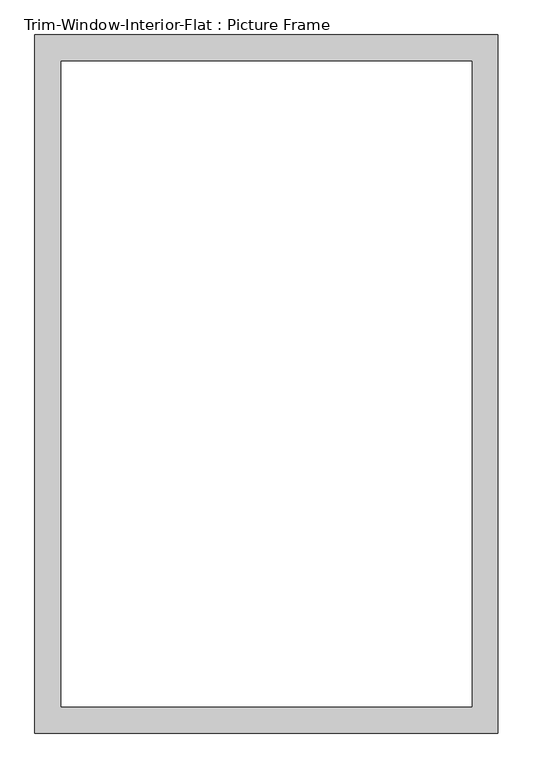
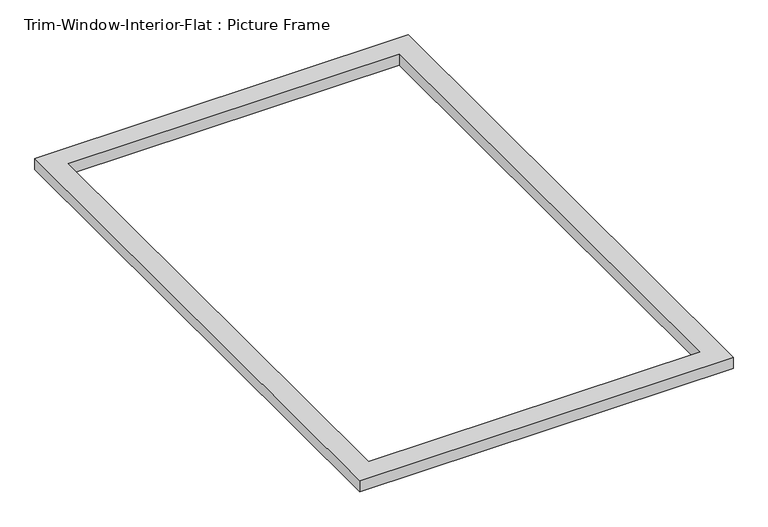
"""IFC4 building model written with IfcOpenShell, lengths in millimetres: proxy geometry, Trim-Window-Interior-Flat : Picture Frame."""

from ifc_helpers import new_model, si_unit, origin, origin_with_axes, place, context, project, spatial, polyline, outline, extrude, source, transform, mapped, element, save


def trim_window_interior_flat_picture_frame_99361138(model_context):
    return source(origin(), model_context, "Body", "SweptSolid", [
        extrude(outline(polyline([(501.65, 44.45), (501.65, -1466.85), (-501.65, -1466.85), (-501.65, 44.45), (501.65, 44.45)]), holes=[polyline([(444.5, -12.7), (-444.5, -12.7), (-444.5, -1409.7), (444.5, -1409.7), (444.5, -12.7)])]), origin_with_axes(), (0.0, 0.0, 1.0), 31.75),
    ])


if __name__ == "__main__":
    model = new_model("IFC4")
    model_context = context("Model", 3, world=origin())
    ifc_project = project(units=[si_unit("LENGTHUNIT", "METRE", prefix="MILLI")], contexts=[model_context])
    site = spatial("IfcSite", under=ifc_project)
    building = spatial("IfcBuilding", under=site)
    placement = place(None, origin())
    trim_window_interior_flat_picture_frame_shape = trim_window_interior_flat_picture_frame_99361138(model_context)
    element("IfcBuildingElementProxy", 1, Name="Trim-Window-Interior-Flat : Picture Frame", ObjectType="Trim-Window-Interior-Flat : Picture Frame", at=placement, inside=building, context=model_context, shape_type="MappedRepresentation", body=[
        mapped(trim_window_interior_flat_picture_frame_shape, transform((0.0, 0.0, 0.0), x_axis=(1.0, 0.0, 0.0), y_axis=(0.0, 1.0, 0.0), z_axis=(0.0, 0.0, 1.0))),
    ])
    save(model, "model.ifc")

# Revit data of these elements
# Type "Trim-Window-Interior-Flat : Picture Frame"
#   Trim Thickness_Picture Frame = 0' - 1 1/4"
#   Trim Width = 0' - 2 1/4"
#   Trim Thickness_with Sill = 0' - 0 3/4"
#   Sill Thickness = 0' - 1 1/4"
#   Opening Width [instance default] = 2' - 0"
#   Opening Height [instance default] = 3' - 0"
#   Default Elevation = 4' - 0"
#   Sill = no
#   Picture Frame = yes
#   Trim Material [instance default] = none
# Element 1 (IfcBuildingElementProxy, "Trim-Window-Interior-Flat : Picture Frame")
#   Opening Width = 3' - 0"
#   Opening Height = 4' - 8"
#   Trim Material = Wood - Stained
#   Materials on its faces: "Wood - Stained"
# Materials
#   "Wood - Stained": class "Wood", colour RGB 224 178 126, transparency 0, Cost = 0
